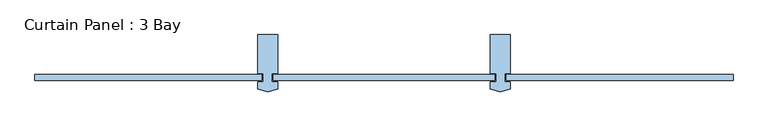
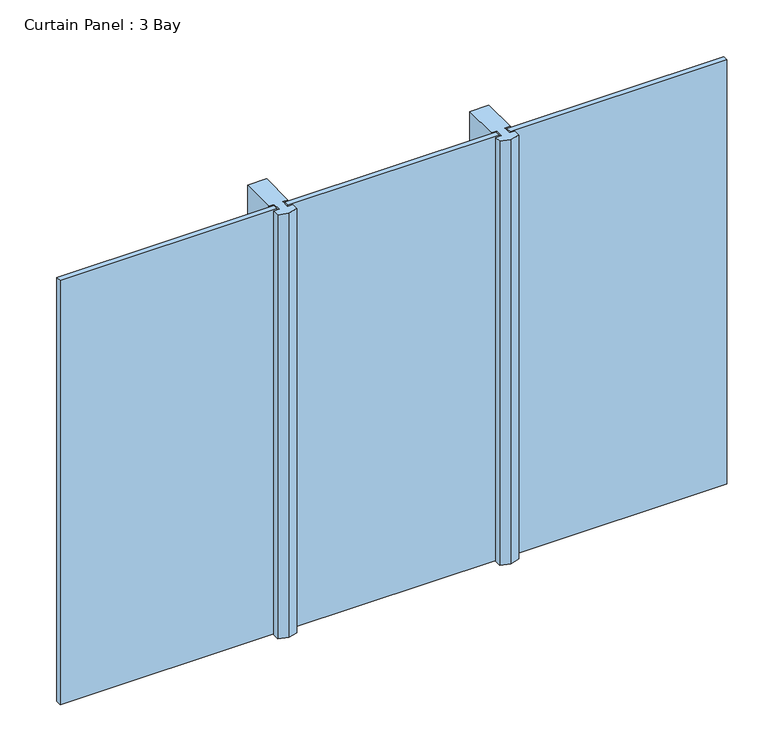
"""IFC4 building model written with IfcOpenShell, lengths in millimetres: window geometry, Curtain Panel : 3 Bay."""

import ifcopenshell
import ifcopenshell.guid

model = None  # the IFC model being written
_history = None  # IfcOwnerHistory: only IFC2X3 demands one
_inside = {}  # id of a spatial element -> (the spatial element, [elements in it])
_under = {}  # id of a project, library or spatial element -> (it, [spatial elements below it])
_declared = {}  # id of a project -> (the project, [libraries it declares])
_typed = {}  # id of a type object -> (the type object, [elements of that type])
_made_of = {}  # id of a material, layer set ... -> (it, [elements and type objects made of it])


def new_model(schema):
    """Start an empty IFC model of exactly this schema.

    Asked for "IFC4X3", IfcOpenShell would pick the latest addendum, in which some entities
    have other attributes; the version numbers below select the first issue.
    IFC2X3 requires an IfcOwnerHistory on every rooted entity: one is made here for all.
    """
    global model, _history
    if schema == "IFC4X3":
        model = ifcopenshell.file(schema_version=(4, 3, 0, 0))
    else:
        model = ifcopenshell.file(schema=schema)
    _inside.clear()
    _under.clear()
    _declared.clear()
    _typed.clear()
    _made_of.clear()
    _history = None
    if model.schema == "IFC2X3":
        org = make("IfcOrganization", Name="unknown")
        user = make(
            "IfcPersonAndOrganization",
            ThePerson=make("IfcPerson", FamilyName="unknown"),
            TheOrganization=org,
        )
        app = make(
            "IfcApplication",
            ApplicationDeveloper=org,
            Version="unknown",
            ApplicationFullName="unknown",
            ApplicationIdentifier="unknown",
        )
        _history = make(
            "IfcOwnerHistory",
            OwningUser=user,
            OwningApplication=app,
            ChangeAction="ADDED",
            CreationDate=0,
        )
    return model


def make(cls, **values):
    """One entity of the class cls with the attributes given. An attribute that is None is left unset."""
    return model.create_entity(
        cls, **{name: value for name, value in values.items() if value is not None}
    )


def rooted(cls, **values):
    """An entity with a GlobalId (a new one), such as an element, a storey or a relation."""
    return make(cls, GlobalId=ifcopenshell.guid.new(), OwnerHistory=_history, **values)


def si_unit(unit_type, name, prefix=None):
    """IfcSIUnit, for example si_unit("LENGTHUNIT", "METRE", prefix="MILLI")."""
    return make("IfcSIUnit", UnitType=unit_type, Prefix=prefix, Name=name)


def assignment(units):
    """IfcUnitAssignment: the units of a project."""
    return None if units is None else make("IfcUnitAssignment", Units=units)


def point(xyz):
    """IfcCartesianPoint."""
    return None if xyz is None else make("IfcCartesianPoint", Coordinates=xyz)


def direction(xyz):
    """IfcDirection."""
    return None if xyz is None else make("IfcDirection", DirectionRatios=xyz)


def frame(location, z_axis=None, x_axis=None):
    """IfcAxis2Placement3D, a coordinate frame: its origin and axes. An axis left out is left unset."""
    return make(
        "IfcAxis2Placement3D",
        Location=point(location),
        Axis=direction(z_axis),
        RefDirection=direction(x_axis),
    )


def origin():
    """The frame at (0, 0, 0) with its axes left unset."""
    return frame((0.0, 0.0, 0.0))


def origin_with_axes():
    """The frame at (0, 0, 0) with the z axis (0, 0, 1) and the x axis (1, 0, 0) written out."""
    return frame((0.0, 0.0, 0.0), z_axis=(0.0, 0.0, 1.0), x_axis=(1.0, 0.0, 0.0))


def place(relative_to, where):
    """IfcLocalPlacement: puts the frame where relative to a parent placement (None: the world)."""
    return make(
        "IfcLocalPlacement", PlacementRelTo=relative_to, RelativePlacement=where
    )


def context(
    kind, dimensions, precision=None, world=None, true_north=None, identifier=None
):
    """IfcGeometricRepresentationContext, for example the 3D "Model" context."""
    return make(
        "IfcGeometricRepresentationContext",
        ContextIdentifier=identifier,
        ContextType=kind,
        CoordinateSpaceDimension=dimensions,
        Precision=precision,
        WorldCoordinateSystem=world,
        TrueNorth=true_north,
    )


def project(units=None, contexts=None):
    """IfcProject with its units and contexts."""
    return rooted(
        "IfcProject",
        Name="project",
        RepresentationContexts=contexts,
        UnitsInContext=assignment(units),
    )


def spatial(cls, under=None, at=None, **own):
    """A site, building, storey or space (cls), placed at a placement, below another one or the project."""
    s = rooted(cls, ObjectPlacement=at, **own)
    if under is not None:
        _under.setdefault(under.id(), (under, []))[1].append(s)
    return s


def polyline(points):
    """IfcPolyline through the points."""
    return make("IfcPolyline", Points=[point(p) for p in points])


def outline(outer, holes=None, kind="AREA"):
    """IfcArbitraryClosedProfileDef: a profile drawn as a closed curve; with holes, ...WithVoids."""
    if holes is None:
        return make("IfcArbitraryClosedProfileDef", ProfileType=kind, OuterCurve=outer)
    return make(
        "IfcArbitraryProfileDefWithVoids",
        ProfileType=kind,
        OuterCurve=outer,
        InnerCurves=holes,
    )


def extrude(swept, where, along, depth):
    """IfcExtrudedAreaSolid: the profile swept, set in the frame where, extruded along a direction by depth."""
    return make(
        "IfcExtrudedAreaSolid",
        SweptArea=swept,
        Position=where,
        ExtrudedDirection=direction(along),
        Depth=depth,
    )


def shape(context_of_items, identifier, shape_type, items):
    """IfcShapeRepresentation: the items that make up one representation, for example the "Body"."""
    return make(
        "IfcShapeRepresentation",
        ContextOfItems=context_of_items,
        RepresentationIdentifier=identifier,
        RepresentationType=shape_type,
        Items=items,
    )


def source(mapping_origin, context_of_items, identifier, shape_type, items):
    """IfcRepresentationMap: a shape defined once, which mapped items show again and again."""
    return make(
        "IfcRepresentationMap",
        MappingOrigin=mapping_origin,
        MappedRepresentation=shape(context_of_items, identifier, shape_type, items),
    )


def transform(
    local_origin,
    x_axis=None,
    y_axis=None,
    z_axis=None,
    scale=None,
    scale2=None,
    scale3=None,
    uniform=True,
):
    """IfcCartesianTransformationOperator3D, or its non-uniform kind. x_axis, y_axis, z_axis: its Axis1, 2, 3."""
    if uniform:
        return make(
            "IfcCartesianTransformationOperator3D",
            Axis1=direction(x_axis),
            Axis2=direction(y_axis),
            LocalOrigin=point(local_origin),
            Scale=scale,
            Axis3=direction(z_axis),
        )
    return make(
        "IfcCartesianTransformationOperator3DnonUniform",
        Axis1=direction(x_axis),
        Axis2=direction(y_axis),
        LocalOrigin=point(local_origin),
        Scale=scale,
        Axis3=direction(z_axis),
        Scale2=scale2,
        Scale3=scale3,
    )


def mapped(mapping_source, mapping_target):
    """IfcMappedItem: shows the shape of a source again, moved by a transform."""
    return make(
        "IfcMappedItem", MappingSource=mapping_source, MappingTarget=mapping_target
    )


def made_of(thing, what):
    """Note that an element or type object is made of a material, layer set ...; save() writes the relation."""
    if what is not None:
        _made_of.setdefault(what.id(), (what, []))[1].append(thing)
    return thing


def element(
    cls,
    number,
    at=None,
    inside=None,
    cuts=None,
    type_object=None,
    material=None,
    context=None,
    identifier="Body",
    shape_type=None,
    held_by="IfcProductDefinitionShape",
    body=None,
    shapes=None,
    **own,
):
    """One element of the class cls, such as IfcWall. Its Tag is "e" and its number.

    at: its placement. inside: the storey or other place that contains it. cuts: it is an
    opening in that element (IfcRelVoidsElement). A single representation is given by context,
    identifier, shape_type and body (its items); several are given by shapes. held_by: the class
    of the entity that holds the representations. save() writes the other relations.
    """
    e = rooted(cls, Tag="e%d" % number, ObjectPlacement=at, **own)
    if body is not None:
        shapes = [shape(context, identifier, shape_type, body)]
    if shapes is not None:
        e.Representation = make(held_by, Representations=shapes)
    if inside is not None:
        _inside.setdefault(inside.id(), (inside, []))[1].append(e)
    if cuts is not None:
        rooted(
            "IfcRelVoidsElement", RelatingBuildingElement=cuts, RelatedOpeningElement=e
        )
    if type_object is not None:
        _typed.setdefault(type_object.id(), (type_object, []))[1].append(e)
    return made_of(e, material)


def aggregate(whole, parts):
    """IfcRelAggregates: a whole, such as a stair, and the parts it consists of."""
    return rooted("IfcRelAggregates", RelatingObject=whole, RelatedObjects=parts)


def save(model, path):
    """Write the relations noted so far, then the file.

    IfcRelAggregates (storeys below a building ...), IfcRelContainedInSpatialStructure (elements
    in a storey), IfcRelDefinesByType, IfcRelAssociatesMaterial and IfcRelDeclares: one each for
    every whole, place, type object, material and project.
    """
    for whole, parts in _under.values():
        aggregate(whole, parts)
    for where, things in _inside.values():
        rooted(
            "IfcRelContainedInSpatialStructure",
            RelatedElements=things,
            RelatingStructure=where,
        )
    for kind, things in _typed.values():
        rooted("IfcRelDefinesByType", RelatedObjects=things, RelatingType=kind)
    for what, things in _made_of.values():
        rooted("IfcRelAssociatesMaterial", RelatedObjects=things, RelatingMaterial=what)
    for by, libraries in _declared.values():
        rooted("IfcRelDeclares", RelatingContext=by, RelatedDefinitions=libraries)
    model.write(path)


def curtain_panel_3_bay_d95054c0(model_context):
    return source(origin(), model_context, "Body", "SweptSolid", [
        extrude(outline(polyline([(-472.0166667, -12.7), (-497.4166667, -12.7), (-497.4166667, -50.8), (-472.0166667, -50.8), (-472.0166667, -82.55), (-516.4666667, -95.25), (-560.9166667, -82.55), (-560.9166667, -50.8), (-535.5166667, -50.8), (-535.5166667, -12.7), (-560.9166667, -12.7), (-560.9166667, 158.75), (-472.0166667, 158.75), (-472.0166667, -12.7)])), origin_with_axes(), (0.0, 0.0, 1.0), 2085.3785982),
        extrude(outline(polyline([(472.0166667, -12.7), (472.0166667, 158.75), (560.9166667, 158.75), (560.9166667, -12.7), (535.5166667, -12.7), (535.5166667, -50.8), (560.9166667, -50.8), (560.9166667, -82.55), (516.4666667, -95.25), (472.0166667, -82.55), (472.0166667, -50.8), (497.4166667, -50.8), (497.4166667, -12.7), (472.0166667, -12.7)])), origin_with_axes(), (0.0, 0.0, 1.0), 2085.3785982),
        extrude(outline(polyline([(-491.0666667, -44.45), (-491.0666667, -19.05), (491.0666667, -19.05), (491.0666667, -44.45), (-491.0666667, -44.45)])), origin_with_axes(), (0.0, 0.0, 1.0), 2085.3785982),
        extrude(outline(polyline([(-1549.4, -44.45), (-1549.4, -19.05), (-541.8666667, -19.05), (-541.8666667, -44.45), (-1549.4, -44.45)])), origin_with_axes(), (0.0, 0.0, 1.0), 2085.3785982),
        extrude(outline(polyline([(541.8666667, -44.45), (541.8666667, -19.05), (1549.4, -19.05), (1549.4, -44.45), (541.8666667, -44.45)])), origin_with_axes(), (0.0, 0.0, 1.0), 2085.3785982),
    ])


if __name__ == "__main__":
    model = new_model("IFC4")
    model_context = context("Model", 3, world=origin())
    ifc_project = project(units=[si_unit("LENGTHUNIT", "METRE", prefix="MILLI")], contexts=[model_context])
    site = spatial("IfcSite", under=ifc_project)
    building = spatial("IfcBuilding", under=site)
    placement = place(None, origin())
    curtain_panel_3_bay_shape = curtain_panel_3_bay_d95054c0(model_context)
    element("IfcWindow", 1, ObjectType="Curtain Panel : 3 Bay", at=placement, inside=building, context=model_context, shape_type="MappedRepresentation", body=[
        mapped(curtain_panel_3_bay_shape, transform((0.0, 0.0, 0.0), x_axis=(1.0, 0.0, 0.0), y_axis=(0.0, 1.0, 0.0), z_axis=(0.0, 0.0, 1.0))),
    ])
    save(model, "model.ifc")

# Revit data of these elements
# Type "Curtain Panel : 3 Bay"
#   Type Mark = "24"
#   Description = "The Aubin Academy Master Series"
#   Offset = 0' - 1 1/4"
# Element 1 (IfcWindow, "Curtain Panel : 3 Bay")
#   Materials on its faces: "Metal - Aluminum", "Glass"
# Materials
#   "Metal - Aluminum": class "Metal", colour RGB 247 247 247, transparency 0
#   "Glass": class "Glass", colour RGB 0 128 192, transparency 0.75, Description = "Soda Lime Glass", Cost = 0
